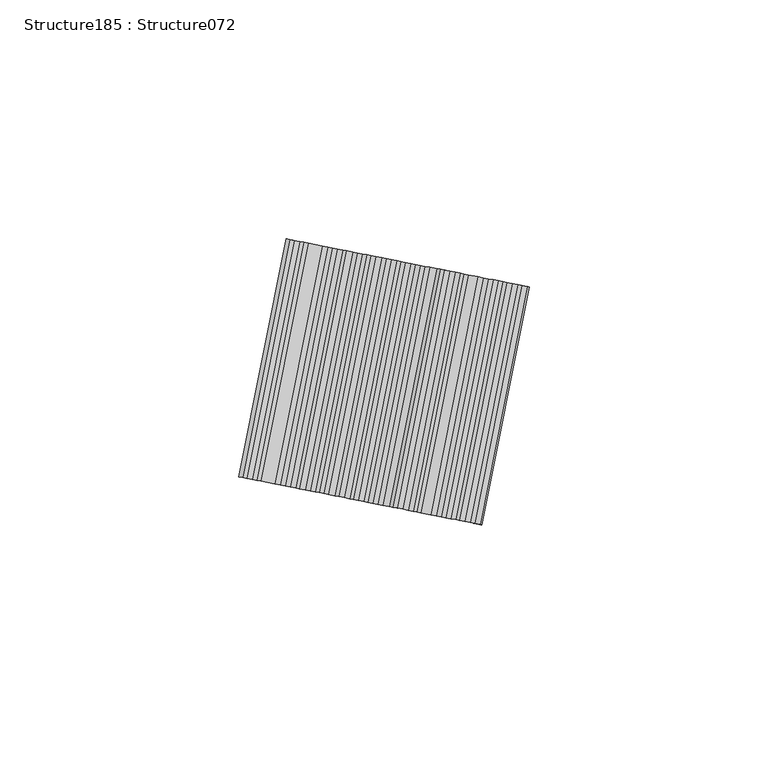
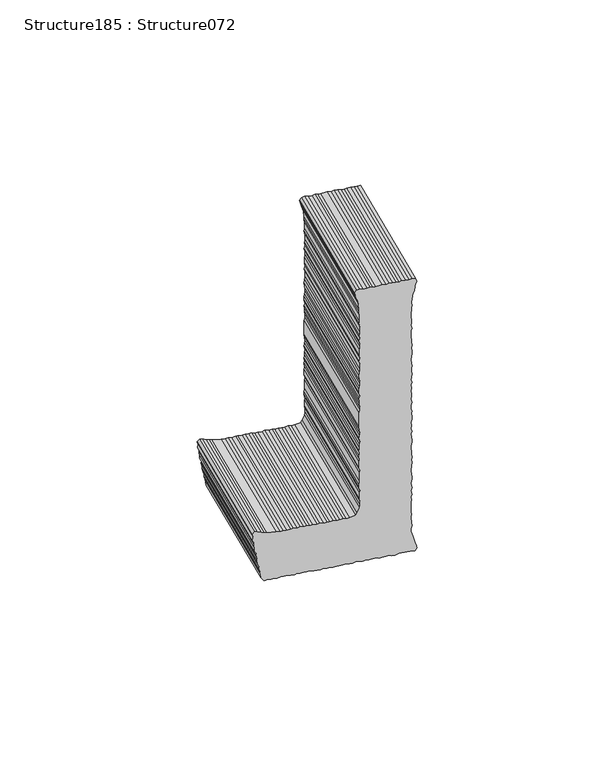
"""IFC4 building model written with IfcOpenShell, lengths in millimetres: proxy geometry, Structure185 : Structure072."""

from ifc_helpers import new_model, si_unit, frame, origin, place, context, project, spatial, polyline, outline, extrude, source, transform, mapped, element, save


def structure185_structure072_a95f546f(model_context):
    return source(origin(), model_context, "Body", "SweptSolid", [
        extrude(outline(polyline([(1.1010061, 0.0), (1.4689097, -0.9240496), (2.4792082, -1.7515268), (2.7518087, -2.5801664), (3.4838749, -3.3169318), (4.2109946, -4.4202642), (4.8547816, -5.0681837), (5.0302244, -5.9878436), (5.85945, -6.6330855), (6.4122109, -7.7361117), (7.0502297, -8.3782259), (7.6890699, -9.3927123), (8.143826, -10.2224378), (8.8758924, -10.9592033), (9.2425421, -11.8819909), (9.8834908, -12.7092928), (10.6147026, -13.6345048), (10.7949436, -15.0991479), (9.6880808, -15.8287721), (9.2244897, -16.6595852), (8.3060733, -17.3900639), (7.8433384, -18.0319274), (6.921992, -18.5772184), (6.2800312, -19.4031836), (5.3550717, -20.1341446), (4.8038967, -21.0519831), (3.9732371, -21.8773446), (3.234126, -22.2415626), (2.5921653, -23.0675279), (1.8523709, -23.8026037), (1.116714, -24.3454696), (0.377172, -25.0802946), (-0.3597719, -26.1827171), (-1.8320409, -27.6455958), (-2.6622696, -28.1003502), (-3.3080959, -29.1122363), (-4.1386759, -29.7554389), (-4.5981296, -30.394042), (-5.5162936, -31.12427), (-5.9828146, -31.7698954), (-6.901231, -32.500374), (-7.7348205, -33.1405478), (-8.2859956, -34.0583863), (-8.9273526, -34.6956526), (-9.8522326, -35.2444548), (-10.5884933, -35.9760195), (-11.2376009, -36.9911659), (-12.2500648, -37.6269932), (-12.7065091, -38.2686253), (-13.6312161, -38.9993354), (-14.4621281, -39.8249477), (-14.8272818, -40.5579514), (-15.6581143, -41.2014047), (-16.4854926, -42.0235059), (-17.2244308, -42.5696321), (-17.6844882, -43.3969341), (-18.4240302, -44.1317592), (-19.5311454, -44.8616342), (-22.4794694, -47.7911534), (-22.9391949, -48.4360457), (-24.1293814, -48.1569864), (-24.7727569, -47.1444983), (-25.1366478, -46.2244872), (-25.6857039, -45.3003612), (-26.325319, -44.2921623), (-27.2382662, -42.4480253), (-27.8762849, -41.805911), (-28.884634, -41.1555672), (-29.6214084, -40.2388918), (-30.9038644, -38.7588973), (-31.7290772, -38.1176937), (-32.2726955, -37.3812796), (-34.655234, -34.9834473), (-35.2993738, -34.5244791), (-36.1206206, -33.5086544), (-36.9448872, -33.0435746), (-37.5872611, -32.0325993), (-38.5015627, -31.4769068), (-39.6011332, -30.0058001), (-40.6962569, -29.2681246), (-41.250009, -28.710818), (-42.0740595, -27.7063062), (-42.7114745, -26.8754932), (-44.0879315, -25.6795071), (-45.0951754, -24.8409692), (-45.6486196, -24.1088007), (-46.3769811, -23.5509355), (-47.2050443, -22.5423853), (-47.8458217, -21.8974946), (-48.3921987, -21.158304), (-49.2153031, -20.3299161), (-50.2221475, -19.6810866), (-50.7731408, -19.1265564), (-51.4163692, -18.3040276), (-52.2386191, -17.2871932), (-53.0618826, -16.8231231), (-53.5204248, -15.9971595), (-54.3499011, -15.3516651), (-55.1681383, -14.3388692), (-56.0809351, -13.784691), (-56.8157601, -13.0451491), (-57.3692044, -12.3129807), (-58.1886039, -11.6634929), (-58.6471461, -10.8375293), (-59.5630441, -9.9157522), (-60.3903203, -9.4476435), (-61.0296846, -8.4396972), (-61.856653, -7.7967268), (-62.5912272, -7.0574373), (-63.0435567, -6.4128979), (-63.8730329, -5.7674036), (-64.6942797, -4.7515788), (-65.5145337, -4.2905375), (-66.0668727, -3.370175), (-66.8025522, -2.8190795), (-67.7117358, -2.0792314), (-68.3592276, -1.2524117), (-68.9997543, -0.6077734), (-69.8221633, 0.0447431), (-71.1040607, 1.6993471), (-71.9332862, 2.344589), (-72.9325047, 3.17505), (-73.5732822, 3.8199407), (-74.2220279, 4.6480224), (-74.9463767, 5.2018493), (-75.7746907, 6.2106518), (-76.325684, 6.765182), (-76.9613436, 7.5942283), (-78.6133206, 9.2568094), (-79.3427873, 9.6264807), (-79.9864151, 10.6387179), (-80.7218438, 11.1895611), (-81.456418, 11.9288506), (-82.1836172, 12.850024), (-83.0097311, 13.6814408), (-83.8389566, 14.3266828), (-84.5697689, 15.0621863), (-85.2043336, 15.5256527), (-85.9426127, 16.4438425), (-86.8517963, 17.1836906), (-88.4134185, 18.3837916), (-89.4232258, 18.6569901), (-90.4299906, 19.4879784), (-91.3468001, 20.046195), (-92.1709197, 20.3213156), (-92.8136915, 21.5225025), (-91.9830319, 22.347864), (-91.2516384, 22.8950207), (-90.5105106, 23.8109934), (-89.679851, 24.636355), (-88.9442735, 24.9970619), (-88.3035668, 25.8242891), (-87.6535565, 26.6497254), (-86.9172959, 27.3812901), (-85.9926683, 27.9298414), (-85.3503756, 28.9382164), (-83.6894873, 30.2183324), (-83.0443442, 30.8593607), (-82.6756569, 31.5958754), (-81.7543105, 32.1411664), (-80.9233985, 32.9667787), (-80.2813583, 33.9749028), (-79.4511296, 34.4296573), (-78.3476967, 34.2444712), (-77.8937709, 33.2338472), (-77.2536767, 32.2180988), (-76.7984173, 31.3883718), (-76.250423, 30.289638), (-74.8746493, 28.7227941), (-74.2338718, 28.0779034), (-73.50266, 27.1526915), (-71.9459846, 25.5860237), (-71.3015939, 25.126803), (-70.5744744, 24.0234706), (-69.1988718, 22.639038), (-68.3756879, 21.992809), (-67.6409424, 21.0711081), (-66.8141453, 20.6105491), (-66.2696034, 19.6909664), (-65.4432388, 18.8592972), (-64.6203056, 18.2133206), (-63.154919, 16.7385276), (-62.5139704, 15.9112257), (-61.5933764, 15.3562677), (-61.2324154, 14.6214443), (-59.7655241, 13.1451369), (-58.9435941, 12.5001699), (-57.9317909, 11.6711782), (-56.6509193, 10.0105392), (-56.0098909, 9.3653961), (-55.1884626, 8.7209339), (-54.4527831, 8.1698384), (-53.6269199, 7.338674), (-52.9905877, 6.3267116), (-52.2513175, 5.9542414), (-51.5241183, 5.0330679), (-50.7923028, 4.2965549), (-50.0575573, 3.374854), (-49.326745, 2.6393506), (-48.408659, 2.0869167), (-44.8386131, -1.5060456), (-44.1984393, -2.3396351), (-43.3739098, -3.3516964), (-42.7358115, -3.8116517), (-41.9063352, -4.4571461), (-41.266241, -5.4728944), (-40.4430571, -6.1191235), (-39.6184479, -6.9490259), (-38.7917304, -7.5917438), (-38.2456042, -8.330682), (-37.5101755, -8.8815251), (-36.6889287, -9.8973498), (-35.8597032, -10.5425918), (-34.3995833, -12.0120844), (-34.0316001, -12.7539751), (-33.2084161, -13.4002041), (-31.0109632, -15.6117626), (-30.0904489, -16.3488794), (-29.4536841, -16.9897316), (-28.7225519, -18.0971024), (-28.0816948, -18.5598342), (-26.5210067, -20.1305405), (-25.9753596, -20.8619292), (-25.0582076, -21.7849684), (-24.3263126, -22.3393226), (-22.5817702, -22.9869897), (-21.7576522, -23.2626134), (-20.0976184, -22.1709438), (-19.2703197, -21.5310014), (-18.7158633, -20.6099027), (-17.7945171, -20.0646117), (-17.1458404, -19.4200723), (-16.4097524, -18.5065995), (-15.5824538, -17.8666572), (-15.1197187, -17.2247938), (-14.1977687, -16.4908039), (-13.555476, -15.4824291), (-12.7254997, -15.0279252), (-11.8945082, -14.0201541), (-11.0672095, -13.3802118), (-10.6038708, -12.5496495), (-9.8682138, -12.0067836), (-9.222467, -11.1770565), (-8.3013731, -10.6320163), (-7.5644292, -9.5295939), (-6.9166085, -9.0740041), (-5.9981922, -8.3435253), (-5.3529695, -7.5203382), (-4.5223896, -6.8771356), (-3.7825156, -5.9599008), (-1.9439861, -3.5753214), (-1.4766346, -2.7487976), (-1.0201108, -1.9250067), (-0.550319, -0.7288888), (0.0, 0.0), (1.1010061, 0.0)])), frame((-2459.0657425, 234956.5008017, 404.7189755), z_axis=(0.1946622229639412, 0.9808703374813295, 0.0), x_axis=(-0.6957954552865148, 0.1380866408928953, -0.7048409494414667)), (0.0, 0.0, 1.0), 50.8),
    ])


if __name__ == "__main__":
    model = new_model("IFC4")
    model_context = context("Model", 3, world=origin())
    ifc_project = project(units=[si_unit("LENGTHUNIT", "METRE", prefix="MILLI")], contexts=[model_context])
    site = spatial("IfcSite", under=ifc_project)
    building = spatial("IfcBuilding", under=site)
    placement = place(None, origin())
    structure185_structure072_shape = structure185_structure072_a95f546f(model_context)
    element("IfcBuildingElementProxy", 1, Name="Structure185 : Structure072", ObjectType="Structure185 : Structure072", at=placement, inside=building, context=model_context, shape_type="MappedRepresentation", body=[
        mapped(structure185_structure072_shape, transform((0.0, 0.0, 0.0), x_axis=(1.0, 0.0, 0.0), y_axis=(0.0, 1.0, 0.0), z_axis=(0.0, 0.0, 1.0))),
    ])
    save(model, "model.ifc")

# Revit data of these elements
# Type "Structure185 : Structure072"
#   NameOverride = "Structure072"
# Element 1 (IfcBuildingElementProxy, "Structure185 : Structure072")
#   Materials on its faces: "BRUSHED ALUMINUM LETTERING"
# Materials
#   "BRUSHED ALUMINUM LETTERING": class "Unassigned", colour RGB 169 181 186, transparency 0, Cost = 0
